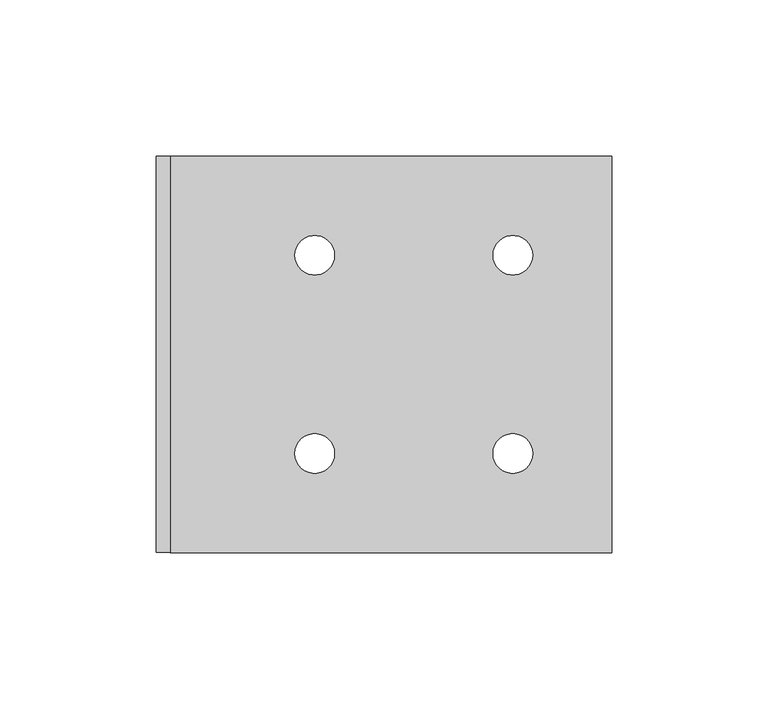
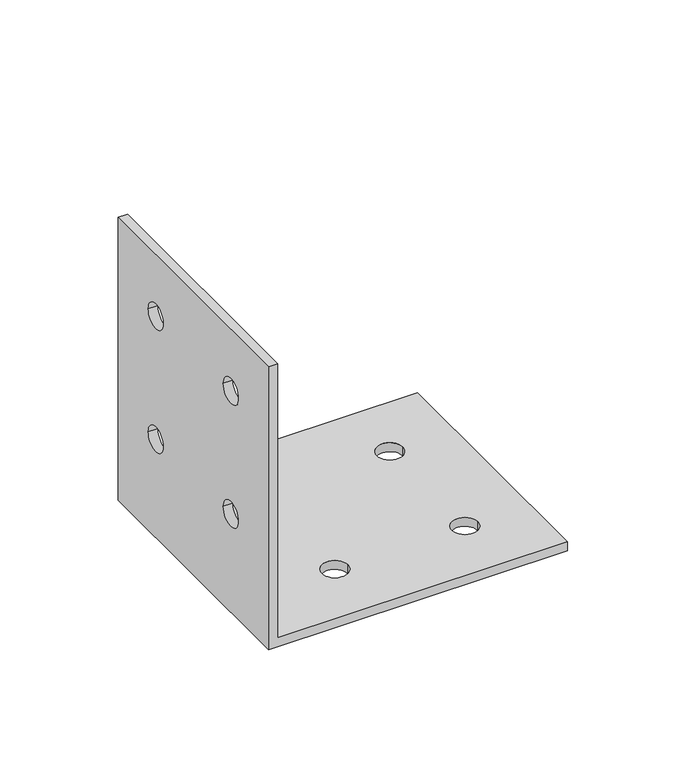
"""IFC4 building model written with IfcOpenShell, lengths in millimetres: fastener geometry."""

import ifcopenshell
import ifcopenshell.guid

model = None  # the IFC model being written
_history = None  # IfcOwnerHistory: only IFC2X3 demands one
_inside = {}  # id of a spatial element -> (the spatial element, [elements in it])
_under = {}  # id of a project, library or spatial element -> (it, [spatial elements below it])
_declared = {}  # id of a project -> (the project, [libraries it declares])
_typed = {}  # id of a type object -> (the type object, [elements of that type])
_made_of = {}  # id of a material, layer set ... -> (it, [elements and type objects made of it])


def new_model(schema):
    """Start an empty IFC model of exactly this schema.

    Asked for "IFC4X3", IfcOpenShell would pick the latest addendum, in which some entities
    have other attributes; the version numbers below select the first issue.
    IFC2X3 requires an IfcOwnerHistory on every rooted entity: one is made here for all.
    """
    global model, _history
    if schema == "IFC4X3":
        model = ifcopenshell.file(schema_version=(4, 3, 0, 0))
    else:
        model = ifcopenshell.file(schema=schema)
    _inside.clear()
    _under.clear()
    _declared.clear()
    _typed.clear()
    _made_of.clear()
    _history = None
    if model.schema == "IFC2X3":
        org = make("IfcOrganization", Name="unknown")
        user = make(
            "IfcPersonAndOrganization",
            ThePerson=make("IfcPerson", FamilyName="unknown"),
            TheOrganization=org,
        )
        app = make(
            "IfcApplication",
            ApplicationDeveloper=org,
            Version="unknown",
            ApplicationFullName="unknown",
            ApplicationIdentifier="unknown",
        )
        _history = make(
            "IfcOwnerHistory",
            OwningUser=user,
            OwningApplication=app,
            ChangeAction="ADDED",
            CreationDate=0,
        )
    return model


def make(cls, **values):
    """One entity of the class cls with the attributes given. An attribute that is None is left unset."""
    return model.create_entity(
        cls, **{name: value for name, value in values.items() if value is not None}
    )


def rooted(cls, **values):
    """An entity with a GlobalId (a new one), such as an element, a storey or a relation."""
    return make(cls, GlobalId=ifcopenshell.guid.new(), OwnerHistory=_history, **values)


def si_unit(unit_type, name, prefix=None):
    """IfcSIUnit, for example si_unit("LENGTHUNIT", "METRE", prefix="MILLI")."""
    return make("IfcSIUnit", UnitType=unit_type, Prefix=prefix, Name=name)


def assignment(units):
    """IfcUnitAssignment: the units of a project."""
    return None if units is None else make("IfcUnitAssignment", Units=units)


def point(xyz):
    """IfcCartesianPoint."""
    return None if xyz is None else make("IfcCartesianPoint", Coordinates=xyz)


def direction(xyz):
    """IfcDirection."""
    return None if xyz is None else make("IfcDirection", DirectionRatios=xyz)


def frame(location, z_axis=None, x_axis=None):
    """IfcAxis2Placement3D, a coordinate frame: its origin and axes. An axis left out is left unset."""
    return make(
        "IfcAxis2Placement3D",
        Location=point(location),
        Axis=direction(z_axis),
        RefDirection=direction(x_axis),
    )


def origin():
    """The frame at (0, 0, 0) with its axes left unset."""
    return frame((0.0, 0.0, 0.0))


def place(relative_to, where):
    """IfcLocalPlacement: puts the frame where relative to a parent placement (None: the world)."""
    return make(
        "IfcLocalPlacement", PlacementRelTo=relative_to, RelativePlacement=where
    )


def context(
    kind, dimensions, precision=None, world=None, true_north=None, identifier=None
):
    """IfcGeometricRepresentationContext, for example the 3D "Model" context."""
    return make(
        "IfcGeometricRepresentationContext",
        ContextIdentifier=identifier,
        ContextType=kind,
        CoordinateSpaceDimension=dimensions,
        Precision=precision,
        WorldCoordinateSystem=world,
        TrueNorth=true_north,
    )


def project(units=None, contexts=None):
    """IfcProject with its units and contexts."""
    return rooted(
        "IfcProject",
        Name="project",
        RepresentationContexts=contexts,
        UnitsInContext=assignment(units),
    )


def spatial(cls, under=None, at=None, **own):
    """A site, building, storey or space (cls), placed at a placement, below another one or the project."""
    s = rooted(cls, ObjectPlacement=at, **own)
    if under is not None:
        _under.setdefault(under.id(), (under, []))[1].append(s)
    return s


def polyline(points):
    """IfcPolyline through the points."""
    return make("IfcPolyline", Points=[point(p) for p in points])


def circle_curve(where, radius):
    """IfcCircle in the frame where."""
    return make("IfcCircle", Position=where, Radius=radius)


def shape(context_of_items, identifier, shape_type, items):
    """IfcShapeRepresentation: the items that make up one representation, for example the "Body"."""
    return make(
        "IfcShapeRepresentation",
        ContextOfItems=context_of_items,
        RepresentationIdentifier=identifier,
        RepresentationType=shape_type,
        Items=items,
    )


def source(mapping_origin, context_of_items, identifier, shape_type, items):
    """IfcRepresentationMap: a shape defined once, which mapped items show again and again."""
    return make(
        "IfcRepresentationMap",
        MappingOrigin=mapping_origin,
        MappedRepresentation=shape(context_of_items, identifier, shape_type, items),
    )


def transform(
    local_origin,
    x_axis=None,
    y_axis=None,
    z_axis=None,
    scale=None,
    scale2=None,
    scale3=None,
    uniform=True,
):
    """IfcCartesianTransformationOperator3D, or its non-uniform kind. x_axis, y_axis, z_axis: its Axis1, 2, 3."""
    if uniform:
        return make(
            "IfcCartesianTransformationOperator3D",
            Axis1=direction(x_axis),
            Axis2=direction(y_axis),
            LocalOrigin=point(local_origin),
            Scale=scale,
            Axis3=direction(z_axis),
        )
    return make(
        "IfcCartesianTransformationOperator3DnonUniform",
        Axis1=direction(x_axis),
        Axis2=direction(y_axis),
        LocalOrigin=point(local_origin),
        Scale=scale,
        Axis3=direction(z_axis),
        Scale2=scale2,
        Scale3=scale3,
    )


def mapped(mapping_source, mapping_target):
    """IfcMappedItem: shows the shape of a source again, moved by a transform."""
    return make(
        "IfcMappedItem", MappingSource=mapping_source, MappingTarget=mapping_target
    )


def made_of(thing, what):
    """Note that an element or type object is made of a material, layer set ...; save() writes the relation."""
    if what is not None:
        _made_of.setdefault(what.id(), (what, []))[1].append(thing)
    return thing


def element(
    cls,
    number,
    at=None,
    inside=None,
    cuts=None,
    type_object=None,
    material=None,
    context=None,
    identifier="Body",
    shape_type=None,
    held_by="IfcProductDefinitionShape",
    body=None,
    shapes=None,
    **own,
):
    """One element of the class cls, such as IfcWall. Its Tag is "e" and its number.

    at: its placement. inside: the storey or other place that contains it. cuts: it is an
    opening in that element (IfcRelVoidsElement). A single representation is given by context,
    identifier, shape_type and body (its items); several are given by shapes. held_by: the class
    of the entity that holds the representations. save() writes the other relations.
    """
    e = rooted(cls, Tag="e%d" % number, ObjectPlacement=at, **own)
    if body is not None:
        shapes = [shape(context, identifier, shape_type, body)]
    if shapes is not None:
        e.Representation = make(held_by, Representations=shapes)
    if inside is not None:
        _inside.setdefault(inside.id(), (inside, []))[1].append(e)
    if cuts is not None:
        rooted(
            "IfcRelVoidsElement", RelatingBuildingElement=cuts, RelatedOpeningElement=e
        )
    if type_object is not None:
        _typed.setdefault(type_object.id(), (type_object, []))[1].append(e)
    return made_of(e, material)


def aggregate(whole, parts):
    """IfcRelAggregates: a whole, such as a stair, and the parts it consists of."""
    return rooted("IfcRelAggregates", RelatingObject=whole, RelatedObjects=parts)


def save(model, path):
    """Write the relations noted so far, then the file.

    IfcRelAggregates (storeys below a building ...), IfcRelContainedInSpatialStructure (elements
    in a storey), IfcRelDefinesByType, IfcRelAssociatesMaterial and IfcRelDeclares: one each for
    every whole, place, type object, material and project.
    """
    for whole, parts in _under.values():
        aggregate(whole, parts)
    for where, things in _inside.values():
        rooted(
            "IfcRelContainedInSpatialStructure",
            RelatedElements=things,
            RelatingStructure=where,
        )
    for kind, things in _typed.values():
        rooted("IfcRelDefinesByType", RelatedObjects=things, RelatingType=kind)
    for what, things in _made_of.values():
        rooted("IfcRelAssociatesMaterial", RelatedObjects=things, RelatingMaterial=what)
    for by, libraries in _declared.values():
        rooted("IfcRelDeclares", RelatingContext=by, RelatedDefinitions=libraries)
    model.write(path)


def plane_surface(at):
    """IfcPlane: the flat surface through the origin of the frame at, square to its z axis."""
    return make("IfcPlane", Position=at)


def revolved_surface(curve, axis_point, axis_direction):
    """IfcSurfaceOfRevolution: the curve turned about the line through axis_point along axis_direction."""
    return make(
        "IfcSurfaceOfRevolution",
        SweptCurve=make("IfcArbitraryOpenProfileDef", ProfileType="CURVE", Curve=curve),
        AxisPosition=make("IfcAxis1Placement", Location=point(axis_point), Axis=direction(axis_direction)),
    )


def advanced_brep(points, edges, surfaces, faces):
    """IfcAdvancedBrep: a solid bounded by faces that lie on surfaces and meet in shared edges.

    An edge is (start, end): straight between two places in points (the first is 0);
    or (start, end, curve); or (start, end, curve, False) where it runs against its curve.
    A face is (place in surfaces, loops), or (place, loops, False) where it looks against
    its surface's normal. A loop lists edges by number (the first is 1), with a minus sign
    where the edge is run from its end to its start. The first loop is the outer one.
    """
    corners = [point(p) for p in points]
    vertices = [make("IfcVertexPoint", VertexGeometry=c) for c in corners]
    made = []
    for start, end, *more in edges:
        made.append(
            make(
                "IfcEdgeCurve",
                EdgeStart=vertices[start],
                EdgeEnd=vertices[end],
                EdgeGeometry=more[0] if more else make("IfcPolyline", Points=[corners[start], corners[end]]),
                SameSense=more[1] if len(more) > 1 else True,
            )
        )
    hull = []
    for where, loops, *sense in faces:
        bounds = []
        for j, loop in enumerate(loops):
            ring = [make("IfcOrientedEdge", EdgeElement=made[abs(k) - 1], Orientation=k > 0) for k in loop]
            bounds.append(
                make(
                    "IfcFaceOuterBound" if j == 0 else "IfcFaceBound",
                    Bound=make("IfcEdgeLoop", EdgeList=ring),
                    Orientation=True,
                )
            )
        hull.append(make("IfcAdvancedFace", Bounds=bounds, FaceSurface=surfaces[where], SameSense=sense[0] if sense else True))
    return make("IfcAdvancedBrep", Outer=make("IfcClosedShell", CfsFaces=hull))


def fastener_faf270b9(model_context):
    return source(origin(), model_context, "Body", "AdvancedBrep", [
        advanced_brep(
        [(4.5640625, 63.5, 146.05), (4.5640625, -63.5, 146.05), (4.5640625, -63.5, 4.5640625), (4.5640625, 63.5, 4.5640625), (4.5640625, -25.4, 50.8), (4.5640625, -38.1, 50.8), (4.5640625, 38.1, 50.8), (4.5640625, 25.4, 50.8), (4.5640625, 38.1, 114.3), (4.5640625, 25.4, 114.3), (4.5640625, -25.4, 114.3), (4.5640625, -38.1, 114.3), (0.0, -63.5, 146.05), (0.0, 63.5, 146.05), (0.0, 63.5, 0.0), (0.0, -63.5, 0.0), (0.0, -38.1, 50.8), (0.0, -25.4, 50.8), (0.0, 25.4, 50.8), (0.0, 38.1, 50.8), (0.0, 25.4, 114.3), (0.0, 38.1, 114.3), (0.0, -38.1, 114.3), (0.0, -25.4, 114.3), (146.05, -63.5, 0.0), (146.05, -63.5, 4.5640625), (146.05, 63.5, 4.5640625), (146.05, 63.5, 0.0), (57.15, -31.75, 4.5640625), (44.45, -31.75, 4.5640625), (120.65, -31.75, 4.5640625), (107.95, -31.75, 4.5640625), (57.15, 31.75, 4.5640625), (44.45, 31.75, 4.5640625), (120.65, 31.75, 4.5640625), (107.95, 31.75, 4.5640625), (44.45, -31.75, 0.0), (57.15, -31.75, 0.0), (107.95, -31.75, 0.0), (120.65, -31.75, 0.0), (44.45, 31.75, 0.0), (57.15, 31.75, 0.0), (107.95, 31.75, 0.0), (120.65, 31.75, 0.0)],
        [
            (0, 1),
            (1, 2),
            (2, 3),
            (3, 0),
            (4, 5, circle_curve(frame((4.5640625, -31.75, 50.8), z_axis=(-1.0, 0.0, 0.0), x_axis=(0.0, 1.0, 0.0)), 6.35)),
            (5, 4, circle_curve(frame((4.5640625, -31.75, 50.8), z_axis=(-1.0, 0.0, 0.0), x_axis=(0.0, 1.0, 0.0)), 6.35)),
            (6, 7, circle_curve(frame((4.5640625, 31.75, 50.8), z_axis=(-1.0, 0.0, 0.0), x_axis=(0.0, 1.0, 0.0)), 6.35)),
            (7, 6, circle_curve(frame((4.5640625, 31.75, 50.8), z_axis=(-1.0, 0.0, 0.0), x_axis=(0.0, 1.0, 0.0)), 6.35)),
            (8, 9, circle_curve(frame((4.5640625, 31.75, 114.3), z_axis=(-1.0, 0.0, 0.0), x_axis=(0.0, 1.0, 0.0)), 6.35)),
            (9, 8, circle_curve(frame((4.5640625, 31.75, 114.3), z_axis=(-1.0, 0.0, 0.0), x_axis=(0.0, 1.0, 0.0)), 6.35)),
            (10, 11, circle_curve(frame((4.5640625, -31.75, 114.3), z_axis=(-1.0, 0.0, 0.0), x_axis=(0.0, 1.0, 0.0)), 6.35)),
            (11, 10, circle_curve(frame((4.5640625, -31.75, 114.3), z_axis=(-1.0, 0.0, 0.0), x_axis=(0.0, 1.0, 0.0)), 6.35)),
            (12, 13),
            (13, 14),
            (14, 15),
            (15, 12),
            (16, 17, circle_curve(frame((0.0, -31.75, 50.8), z_axis=(1.0, 0.0, 0.0), x_axis=(0.0, 1.0, 0.0)), 6.35)),
            (17, 16, circle_curve(frame((0.0, -31.75, 50.8), z_axis=(1.0, 0.0, 0.0), x_axis=(0.0, 1.0, 0.0)), 6.35)),
            (18, 19, circle_curve(frame((0.0, 31.75, 50.8), z_axis=(1.0, 0.0, 0.0), x_axis=(0.0, 1.0, 0.0)), 6.35)),
            (19, 18, circle_curve(frame((0.0, 31.75, 50.8), z_axis=(1.0, 0.0, 0.0), x_axis=(0.0, 1.0, 0.0)), 6.35)),
            (20, 21, circle_curve(frame((0.0, 31.75, 114.3), z_axis=(1.0, 0.0, 0.0), x_axis=(0.0, 1.0, 0.0)), 6.35)),
            (21, 20, circle_curve(frame((0.0, 31.75, 114.3), z_axis=(1.0, 0.0, 0.0), x_axis=(0.0, 1.0, 0.0)), 6.35)),
            (22, 23, circle_curve(frame((0.0, -31.75, 114.3), z_axis=(1.0, 0.0, 0.0), x_axis=(0.0, 1.0, 0.0)), 6.35)),
            (23, 22, circle_curve(frame((0.0, -31.75, 114.3), z_axis=(1.0, 0.0, 0.0), x_axis=(0.0, 1.0, 0.0)), 6.35)),
            (0, 13),
            (12, 1),
            (15, 24),
            (24, 25),
            (25, 2),
            (3, 26),
            (26, 27),
            (27, 14),
            (25, 26),
            (28, 29, circle_curve(frame((50.8, -31.75, 4.5640625), z_axis=(0.0, 0.0, -1.0), x_axis=(1.0, 0.0, 0.0)), 6.35)),
            (29, 28, circle_curve(frame((50.8, -31.75, 4.5640625), z_axis=(0.0, 0.0, -1.0), x_axis=(1.0, 0.0, 0.0)), 6.35)),
            (30, 31, circle_curve(frame((114.3, -31.75, 4.5640625), z_axis=(0.0, 0.0, -1.0), x_axis=(1.0, 0.0, 0.0)), 6.35)),
            (31, 30, circle_curve(frame((114.3, -31.75, 4.5640625), z_axis=(0.0, 0.0, -1.0), x_axis=(1.0, 0.0, 0.0)), 6.35)),
            (32, 33, circle_curve(frame((50.8, 31.75, 4.5640625), z_axis=(0.0, 0.0, -1.0), x_axis=(1.0, 0.0, 0.0)), 6.35)),
            (33, 32, circle_curve(frame((50.8, 31.75, 4.5640625), z_axis=(0.0, 0.0, -1.0), x_axis=(1.0, 0.0, 0.0)), 6.35)),
            (34, 35, circle_curve(frame((114.3, 31.75, 4.5640625), z_axis=(0.0, 0.0, -1.0), x_axis=(1.0, 0.0, 0.0)), 6.35)),
            (35, 34, circle_curve(frame((114.3, 31.75, 4.5640625), z_axis=(0.0, 0.0, -1.0), x_axis=(1.0, 0.0, 0.0)), 6.35)),
            (27, 24),
            (36, 37, circle_curve(frame((50.8, -31.75, 0.0), z_axis=(0.0, 0.0, 1.0), x_axis=(1.0, 0.0, 0.0)), 6.35)),
            (37, 36, circle_curve(frame((50.8, -31.75, 0.0), z_axis=(0.0, 0.0, 1.0), x_axis=(1.0, 0.0, 0.0)), 6.35)),
            (38, 39, circle_curve(frame((114.3, -31.75, 0.0), z_axis=(0.0, 0.0, 1.0), x_axis=(1.0, 0.0, 0.0)), 6.35)),
            (39, 38, circle_curve(frame((114.3, -31.75, 0.0), z_axis=(0.0, 0.0, 1.0), x_axis=(1.0, 0.0, 0.0)), 6.35)),
            (40, 41, circle_curve(frame((50.8, 31.75, 0.0), z_axis=(0.0, 0.0, 1.0), x_axis=(1.0, 0.0, 0.0)), 6.35)),
            (41, 40, circle_curve(frame((50.8, 31.75, 0.0), z_axis=(0.0, 0.0, 1.0), x_axis=(1.0, 0.0, 0.0)), 6.35)),
            (42, 43, circle_curve(frame((114.3, 31.75, 0.0), z_axis=(0.0, 0.0, 1.0), x_axis=(1.0, 0.0, 0.0)), 6.35)),
            (43, 42, circle_curve(frame((114.3, 31.75, 0.0), z_axis=(0.0, 0.0, 1.0), x_axis=(1.0, 0.0, 0.0)), 6.35)),
            (28, 37),
            (36, 29),
            (38, 31),
            (30, 39),
            (40, 33),
            (32, 41),
            (42, 35),
            (34, 43),
            (4, 17),
            (16, 5),
            (18, 7),
            (6, 19),
            (20, 9),
            (8, 21),
            (22, 11),
            (10, 23),
        ],
        [
            plane_surface(frame((4.5640625, -63.5, 146.05), z_axis=(1.0, 0.0, 0.0), x_axis=(0.0, -1.0, 0.0))),
            plane_surface(frame((0.0, -63.5, 146.05), z_axis=(-1.0, 0.0, 0.0), x_axis=(0.0, 1.0, 0.0))),
            plane_surface(frame((4.5640625, 63.5, 146.05), z_axis=(0.0, 0.0, 1.0), x_axis=(-1.0, 0.0, 0.0))),
            plane_surface(frame((4.5640625, -63.5, 146.05), z_axis=(0.0, -1.0, 0.0), x_axis=(-1.0, 0.0, 0.0))),
            plane_surface(frame((4.5640625, 63.5, 4.5640625), z_axis=(0.0, 1.0, 0.0), x_axis=(-1.0, 0.0, 0.0))),
            plane_surface(frame((0.0, 63.5, 4.5640625), z_axis=(0.0, 0.0, 1.0), x_axis=(-1.0, 0.0, 0.0))),
            plane_surface(frame((0.0, 63.5, 0.0), z_axis=(0.0, 0.0, -1.0), x_axis=(1.0, 0.0, 0.0))),
            plane_surface(frame((146.05, -63.5, 4.5640625), z_axis=(1.0, 0.0, 0.0), x_axis=(0.0, 0.0, -1.0))),
            revolved_surface(polyline([(57.15, -31.75, 4.5640625), (57.15, -31.75, 0.0)]), (50.8, -31.75, 0.0), (0.0, 0.0, 1.0)),
            revolved_surface(polyline([(120.64999999999999, -31.75, 4.5640625), (120.64999999999999, -31.75, 0.0)]), (114.3, -31.75, 0.0), (0.0, 0.0, 1.0)),
            revolved_surface(polyline([(57.15, 31.75, 4.5640625), (57.15, 31.75, 0.0)]), (50.8, 31.75, 0.0), (0.0, 0.0, 1.0)),
            revolved_surface(polyline([(120.64999999999999, 31.75, 4.5640625), (120.64999999999999, 31.75, 0.0)]), (114.3, 31.75, 0.0), (0.0, 0.0, 1.0)),
            revolved_surface(polyline([(4.5640625, -25.4, 50.8), (0.0, -25.4, 50.8)]), (0.0, -31.75, 50.8), (1.0, 0.0, 0.0)),
            revolved_surface(polyline([(4.5640625, 38.1, 50.8), (0.0, 38.1, 50.8)]), (0.0, 31.75, 50.8), (1.0, 0.0, 0.0)),
            revolved_surface(polyline([(4.5640625, 38.1, 114.3), (0.0, 38.1, 114.3)]), (0.0, 31.75, 114.3), (1.0, 0.0, 0.0)),
            revolved_surface(polyline([(4.5640625, -25.4, 114.3), (0.0, -25.4, 114.3)]), (0.0, -31.75, 114.3), (1.0, 0.0, 0.0)),
        ],
        [
            (0, [[1, 2, 3, 4], [5, 6], [7, 8], [9, 10], [11, 12]]),
            (1, [[13, 14, 15, 16], [17, 18], [19, 20], [21, 22], [23, 24]]),
            (2, [[-1, 25, -13, 26]]),
            (3, [[-2, -26, -16, 27, 28, 29]]),
            (4, [[-4, 30, 31, 32, -14, -25]]),
            (5, [[33, -30, -3, -29], [34, 35], [36, 37], [38, 39], [40, 41]]),
            (6, [[42, -27, -15, -32], [43, 44], [45, 46], [47, 48], [49, 50]]),
            (7, [[-33, -28, -42, -31]]),
            (8, [[51, -43, 52, -34]]),
            (8, [[-51, -35, -52, -44]]),
            (9, [[53, -36, 54, -45]]),
            (9, [[-53, -46, -54, -37]]),
            (10, [[55, -38, 56, -47]]),
            (10, [[-55, -48, -56, -39]]),
            (11, [[57, -40, 58, -49]]),
            (11, [[-57, -50, -58, -41]]),
            (12, [[59, -17, 60, -5]]),
            (12, [[-59, -6, -60, -18]]),
            (13, [[61, -7, 62, -19]]),
            (13, [[-61, -20, -62, -8]]),
            (14, [[63, -9, 64, -21]]),
            (14, [[-63, -22, -64, -10]]),
            (15, [[65, -11, 66, -23]]),
            (15, [[-65, -24, -66, -12]]),
        ],
    ),
    ])


if __name__ == "__main__":
    model = new_model("IFC4")
    model_context = context("Model", 3, world=origin())
    ifc_project = project(units=[si_unit("LENGTHUNIT", "METRE", prefix="MILLI")], contexts=[model_context])
    site = spatial("IfcSite", under=ifc_project)
    building = spatial("IfcBuilding", under=site)
    placement = place(None, origin())
    fastener_shape = fastener_faf270b9(model_context)
    element("IfcFastener", 1, ObjectType="060523 - W_P_C - Fastenings - Simpson - HLGPC Heavy Angles and Gussets NO BOLTS : SIMPSON -HL55 - 5 X 5.75 - .5\" BOLT - HDG", at=placement, inside=building, context=model_context, shape_type="MappedRepresentation", body=[
        mapped(fastener_shape, transform((0.0, 0.0, 0.0), x_axis=(1.0, 0.0, 0.0), y_axis=(0.0, 1.0, 0.0), z_axis=(0.0, 0.0, 1.0))),
    ])
    save(model, "model.ifc")

# Revit data of these elements
# Type "060523 - W_P_C - Fastenings - Simpson - HLGPC Heavy Angles and Gussets NO BOLTS : SIMPSON -HL55 - 5 X 5.75 - .5\" BOLT - HDG"
#   URL = "https://www.strongtie.com/classiccollection_architecturalproductsgroup/hlpc-hlgpc_productgroup_wcc/p/hlpc.hlgpc"
#   L = 0' - 5"
#   Hole Radius = 0' - 0 1/4"
#   D4 = 0' - 2 1/2"
#   D2 = 0' - 2 1/2"
#   D1 = 0' - 1 1/4"
#   D3 = 0' - 2"
#   Ga. = 0' - 0 23/128"
#   W1 & W2 = 0' - 5 3/4"
#   Default Elevation = 4' - 0"
#   Bolt Visibility - 3B = no
#   Bolt Visibility - 3A = no
#   Bolt Visibility - 2B = yes
#   Bolt Visibility - 2A = yes
#   Bolt Visibility - 1B = yes
#   Bolt Visibility - 1A = yes
#   Bolt Visibility = yes
#   Bolt Size = element 1549524
# Element 1 (IfcFastener, "060523 - W_P_C - Fastenings - Simpson - HLGPC Heavy Angles and Gussets NO BOLTS : SIMPSON -HL55 - 5 X 5.75 - .5\" BOLT - HDG")
#   Materials on its faces: "SIMPSON -HL55 - 5 X 5.75 - .5\" BOLT (3 GA - RAW STEEL - NO FINISH)"
# Materials
#   "SIMPSON -HL55 - 5 X 5.75 - .5\" BOLT (3 GA - RAW STEEL - NO FINISH)": class "Generic", colour RGB 120 120 120, transparency 0, Cost = 0
